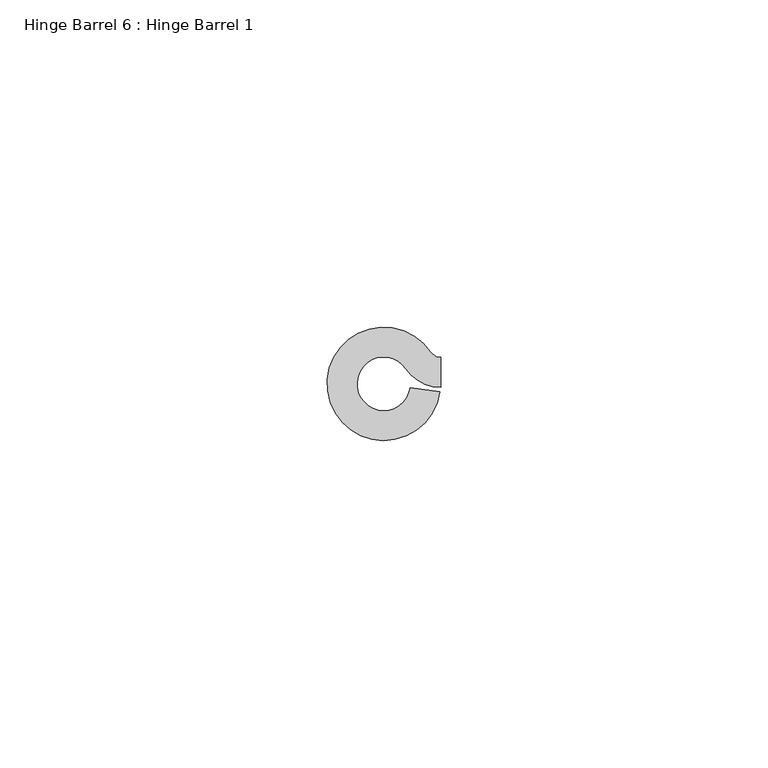
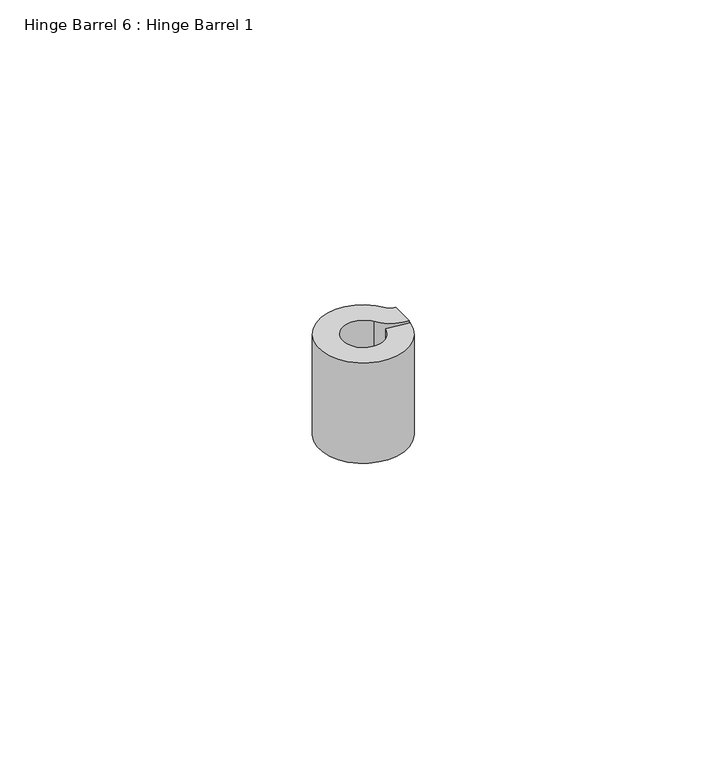
"""IFC4 building model written with IfcOpenShell, lengths in millimetres: proxy geometry, Hinge Barrel 6 : Hinge Barrel 1."""

from ifc_helpers import new_model, si_unit, point, frame, frame_2d, origin, place, context, project, spatial, polyline, circle_curve, trimmed, segment, composite_curve, outline, extrude, source, transform, mapped, element, save


def hinge_barrel_6_hinge_barrel_1_f6209b09(model_context):
    return source(origin(), model_context, "Body", "SweptSolid", [
        extrude(outline(composite_curve([segment(trimmed(circle_curve(frame_2d((587319.1320739, -531776.6049841)), 4.0894), [point((587322.5194669, -531774.3139665))], [point((587323.1821338, -531777.1708529))], True, "CARTESIAN"), True, "CONTINUOUS"), segment(polyline([(587323.1821338, -531777.1708529), (587327.7022899, -531777.8024028)]), True, "CONTINUOUS"), segment(trimmed(circle_curve(frame_2d((587319.1320739, -531776.6049841)), 8.6534625), [point((587327.7022899, -531777.8024028))], [point((587326.3000393, -531771.7570273))], False, "CARTESIAN"), True, "CONTINUOUS"), segment(trimmed(circle_curve(frame_2d((587327.8245257, -531770.7259615)), 1.8404226), [point((587326.3000393, -531771.7570273))], [point((587327.8245257, -531772.5663841))], True, "CARTESIAN"), True, "CONTINUOUS"), segment(polyline([(587327.8245257, -531772.5663841), (587327.8245257, -531777.1304466)]), True, "CONTINUOUS"), segment(trimmed(circle_curve(frame_2d((587327.8245257, -531770.7259615)), 6.4044851), [point((587327.8245257, -531777.1304466))], [point((587322.5194669, -531774.3139665))], False, "CARTESIAN"), True, "CONTINUOUS")], self_intersect=False)), frame((0.0, 0.0, 438.15), z_axis=(0.0, 0.0, 1.0), x_axis=(1.0, 0.0, 0.0)), (0.0, 0.0, 1.0), 20.8359375),
    ])


if __name__ == "__main__":
    model = new_model("IFC4")
    model_context = context("Model", 3, world=origin())
    ifc_project = project(units=[si_unit("LENGTHUNIT", "METRE", prefix="MILLI")], contexts=[model_context])
    site = spatial("IfcSite", under=ifc_project)
    building = spatial("IfcBuilding", under=site)
    placement = place(None, origin())
    hinge_barrel_6_hinge_barrel_1_shape = hinge_barrel_6_hinge_barrel_1_f6209b09(model_context)
    element("IfcBuildingElementProxy", 1, Name="Hinge Barrel 6 : Hinge Barrel 1", ObjectType="Hinge Barrel 6 : Hinge Barrel 1", at=placement, inside=building, context=model_context, shape_type="MappedRepresentation", body=[
        mapped(hinge_barrel_6_hinge_barrel_1_shape, transform((0.0, 0.0, 0.0), x_axis=(1.0, 0.0, 0.0), y_axis=(0.0, 1.0, 0.0), z_axis=(0.0, 0.0, 1.0))),
    ])
    save(model, "model.ifc")

# Revit data of these elements
# Element 1 (IfcBuildingElementProxy, "Hinge Barrel 6 : Hinge Barrel 1")
#   Materials on its faces: "6\"X6\" WELD-ON STL BUTT HINGE"
# Materials
#   "6\"X6\" WELD-ON STL BUTT HINGE": class "Metal", colour RGB 189 187 185, transparency 0, Description = "Carbon steel", Cost = 0
